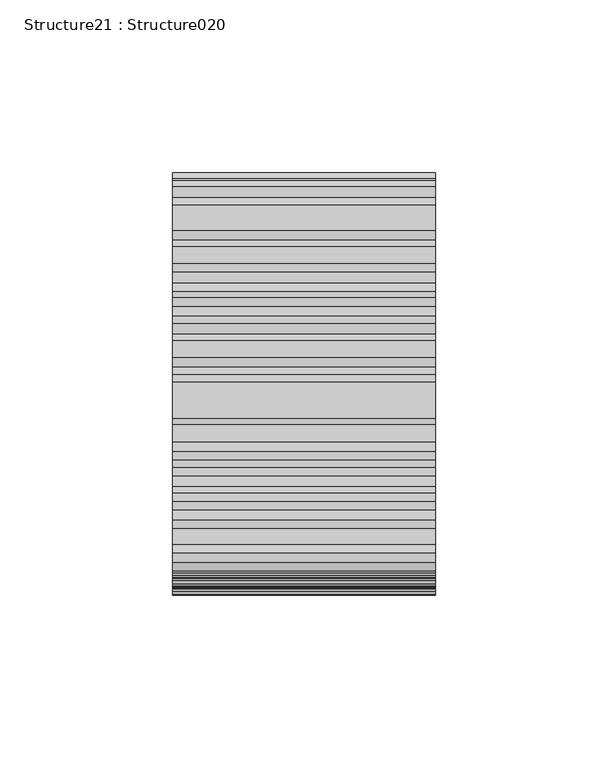
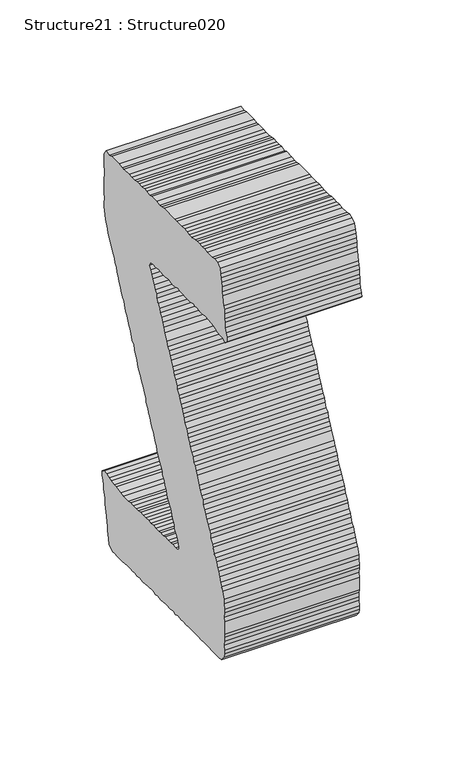
"""IFC4 building model written with IfcOpenShell, lengths in millimetres: proxy geometry, Structure21 : Structure020."""

import ifcopenshell
import ifcopenshell.guid

model = None  # the IFC model being written
_history = None  # IfcOwnerHistory: only IFC2X3 demands one
_inside = {}  # id of a spatial element -> (the spatial element, [elements in it])
_under = {}  # id of a project, library or spatial element -> (it, [spatial elements below it])
_declared = {}  # id of a project -> (the project, [libraries it declares])
_typed = {}  # id of a type object -> (the type object, [elements of that type])
_made_of = {}  # id of a material, layer set ... -> (it, [elements and type objects made of it])


def new_model(schema):
    """Start an empty IFC model of exactly this schema.

    Asked for "IFC4X3", IfcOpenShell would pick the latest addendum, in which some entities
    have other attributes; the version numbers below select the first issue.
    IFC2X3 requires an IfcOwnerHistory on every rooted entity: one is made here for all.
    """
    global model, _history
    if schema == "IFC4X3":
        model = ifcopenshell.file(schema_version=(4, 3, 0, 0))
    else:
        model = ifcopenshell.file(schema=schema)
    _inside.clear()
    _under.clear()
    _declared.clear()
    _typed.clear()
    _made_of.clear()
    _history = None
    if model.schema == "IFC2X3":
        org = make("IfcOrganization", Name="unknown")
        user = make(
            "IfcPersonAndOrganization",
            ThePerson=make("IfcPerson", FamilyName="unknown"),
            TheOrganization=org,
        )
        app = make(
            "IfcApplication",
            ApplicationDeveloper=org,
            Version="unknown",
            ApplicationFullName="unknown",
            ApplicationIdentifier="unknown",
        )
        _history = make(
            "IfcOwnerHistory",
            OwningUser=user,
            OwningApplication=app,
            ChangeAction="ADDED",
            CreationDate=0,
        )
    return model


def make(cls, **values):
    """One entity of the class cls with the attributes given. An attribute that is None is left unset."""
    return model.create_entity(
        cls, **{name: value for name, value in values.items() if value is not None}
    )


def rooted(cls, **values):
    """An entity with a GlobalId (a new one), such as an element, a storey or a relation."""
    return make(cls, GlobalId=ifcopenshell.guid.new(), OwnerHistory=_history, **values)


def si_unit(unit_type, name, prefix=None):
    """IfcSIUnit, for example si_unit("LENGTHUNIT", "METRE", prefix="MILLI")."""
    return make("IfcSIUnit", UnitType=unit_type, Prefix=prefix, Name=name)


def assignment(units):
    """IfcUnitAssignment: the units of a project."""
    return None if units is None else make("IfcUnitAssignment", Units=units)


def point(xyz):
    """IfcCartesianPoint."""
    return None if xyz is None else make("IfcCartesianPoint", Coordinates=xyz)


def direction(xyz):
    """IfcDirection."""
    return None if xyz is None else make("IfcDirection", DirectionRatios=xyz)


def frame(location, z_axis=None, x_axis=None):
    """IfcAxis2Placement3D, a coordinate frame: its origin and axes. An axis left out is left unset."""
    return make(
        "IfcAxis2Placement3D",
        Location=point(location),
        Axis=direction(z_axis),
        RefDirection=direction(x_axis),
    )


def origin():
    """The frame at (0, 0, 0) with its axes left unset."""
    return frame((0.0, 0.0, 0.0))


def place(relative_to, where):
    """IfcLocalPlacement: puts the frame where relative to a parent placement (None: the world)."""
    return make(
        "IfcLocalPlacement", PlacementRelTo=relative_to, RelativePlacement=where
    )


def context(
    kind, dimensions, precision=None, world=None, true_north=None, identifier=None
):
    """IfcGeometricRepresentationContext, for example the 3D "Model" context."""
    return make(
        "IfcGeometricRepresentationContext",
        ContextIdentifier=identifier,
        ContextType=kind,
        CoordinateSpaceDimension=dimensions,
        Precision=precision,
        WorldCoordinateSystem=world,
        TrueNorth=true_north,
    )


def project(units=None, contexts=None):
    """IfcProject with its units and contexts."""
    return rooted(
        "IfcProject",
        Name="project",
        RepresentationContexts=contexts,
        UnitsInContext=assignment(units),
    )


def spatial(cls, under=None, at=None, **own):
    """A site, building, storey or space (cls), placed at a placement, below another one or the project."""
    s = rooted(cls, ObjectPlacement=at, **own)
    if under is not None:
        _under.setdefault(under.id(), (under, []))[1].append(s)
    return s


def polyline(points):
    """IfcPolyline through the points."""
    return make("IfcPolyline", Points=[point(p) for p in points])


def outline(outer, holes=None, kind="AREA"):
    """IfcArbitraryClosedProfileDef: a profile drawn as a closed curve; with holes, ...WithVoids."""
    if holes is None:
        return make("IfcArbitraryClosedProfileDef", ProfileType=kind, OuterCurve=outer)
    return make(
        "IfcArbitraryProfileDefWithVoids",
        ProfileType=kind,
        OuterCurve=outer,
        InnerCurves=holes,
    )


def extrude(swept, where, along, depth):
    """IfcExtrudedAreaSolid: the profile swept, set in the frame where, extruded along a direction by depth."""
    return make(
        "IfcExtrudedAreaSolid",
        SweptArea=swept,
        Position=where,
        ExtrudedDirection=direction(along),
        Depth=depth,
    )


def shape(context_of_items, identifier, shape_type, items):
    """IfcShapeRepresentation: the items that make up one representation, for example the "Body"."""
    return make(
        "IfcShapeRepresentation",
        ContextOfItems=context_of_items,
        RepresentationIdentifier=identifier,
        RepresentationType=shape_type,
        Items=items,
    )


def source(mapping_origin, context_of_items, identifier, shape_type, items):
    """IfcRepresentationMap: a shape defined once, which mapped items show again and again."""
    return make(
        "IfcRepresentationMap",
        MappingOrigin=mapping_origin,
        MappedRepresentation=shape(context_of_items, identifier, shape_type, items),
    )


def transform(
    local_origin,
    x_axis=None,
    y_axis=None,
    z_axis=None,
    scale=None,
    scale2=None,
    scale3=None,
    uniform=True,
):
    """IfcCartesianTransformationOperator3D, or its non-uniform kind. x_axis, y_axis, z_axis: its Axis1, 2, 3."""
    if uniform:
        return make(
            "IfcCartesianTransformationOperator3D",
            Axis1=direction(x_axis),
            Axis2=direction(y_axis),
            LocalOrigin=point(local_origin),
            Scale=scale,
            Axis3=direction(z_axis),
        )
    return make(
        "IfcCartesianTransformationOperator3DnonUniform",
        Axis1=direction(x_axis),
        Axis2=direction(y_axis),
        LocalOrigin=point(local_origin),
        Scale=scale,
        Axis3=direction(z_axis),
        Scale2=scale2,
        Scale3=scale3,
    )


def mapped(mapping_source, mapping_target):
    """IfcMappedItem: shows the shape of a source again, moved by a transform."""
    return make(
        "IfcMappedItem", MappingSource=mapping_source, MappingTarget=mapping_target
    )


def made_of(thing, what):
    """Note that an element or type object is made of a material, layer set ...; save() writes the relation."""
    if what is not None:
        _made_of.setdefault(what.id(), (what, []))[1].append(thing)
    return thing


def element(
    cls,
    number,
    at=None,
    inside=None,
    cuts=None,
    type_object=None,
    material=None,
    context=None,
    identifier="Body",
    shape_type=None,
    held_by="IfcProductDefinitionShape",
    body=None,
    shapes=None,
    **own,
):
    """One element of the class cls, such as IfcWall. Its Tag is "e" and its number.

    at: its placement. inside: the storey or other place that contains it. cuts: it is an
    opening in that element (IfcRelVoidsElement). A single representation is given by context,
    identifier, shape_type and body (its items); several are given by shapes. held_by: the class
    of the entity that holds the representations. save() writes the other relations.
    """
    e = rooted(cls, Tag="e%d" % number, ObjectPlacement=at, **own)
    if body is not None:
        shapes = [shape(context, identifier, shape_type, body)]
    if shapes is not None:
        e.Representation = make(held_by, Representations=shapes)
    if inside is not None:
        _inside.setdefault(inside.id(), (inside, []))[1].append(e)
    if cuts is not None:
        rooted(
            "IfcRelVoidsElement", RelatingBuildingElement=cuts, RelatedOpeningElement=e
        )
    if type_object is not None:
        _typed.setdefault(type_object.id(), (type_object, []))[1].append(e)
    return made_of(e, material)


def aggregate(whole, parts):
    """IfcRelAggregates: a whole, such as a stair, and the parts it consists of."""
    return rooted("IfcRelAggregates", RelatingObject=whole, RelatedObjects=parts)


def save(model, path):
    """Write the relations noted so far, then the file.

    IfcRelAggregates (storeys below a building ...), IfcRelContainedInSpatialStructure (elements
    in a storey), IfcRelDefinesByType, IfcRelAssociatesMaterial and IfcRelDeclares: one each for
    every whole, place, type object, material and project.
    """
    for whole, parts in _under.values():
        aggregate(whole, parts)
    for where, things in _inside.values():
        rooted(
            "IfcRelContainedInSpatialStructure",
            RelatedElements=things,
            RelatingStructure=where,
        )
    for kind, things in _typed.values():
        rooted("IfcRelDefinesByType", RelatedObjects=things, RelatingType=kind)
    for what, things in _made_of.values():
        rooted("IfcRelAssociatesMaterial", RelatedObjects=things, RelatingMaterial=what)
    for by, libraries in _declared.values():
        rooted("IfcRelDeclares", RelatingContext=by, RelatedDefinitions=libraries)
    model.write(path)


def structure21_structure020_0772803a(model_context):
    return source(origin(), model_context, "Body", "SweptSolid", [
        extrude(outline(polyline([(2.4918624, 0.0), (3.6053821, -2.5777483), (4.2923985, -5.0322892), (4.9784696, -7.4834674), (6.2051097, -9.6307181), (6.786362, -12.5115543), (7.588599, -14.5461058), (8.7040111, -17.1169191), (9.3907122, -19.5726158), (10.0484988, -21.3355177), (10.7366711, -23.790374), (11.6968084, -26.099624), (12.9590891, -28.9309487), (14.0327669, -30.8104368), (14.728504, -33.2717039), (15.5358903, -35.3033137), (16.5218964, -38.2914876), (14.6515494, -41.8644896), (12.6100629, -42.6648342), (10.8881597, -44.0143665), (6.0551905, -46.7752522), (1.4453072, -48.6935312), (-0.4349165, -49.7676293), (-2.6987534, -51.4101604), (-5.0008586, -52.3759729), (-6.3008802, -53.8337906), (-8.7605703, -54.5237486), (-11.1382631, -56.5971976), (-16.0151735, -58.6680188), (-20.0426478, -60.9687569), (-21.8811372, -62.7341801), (-24.0738003, -63.2715961), (-26.1837303, -65.1920828), (-28.5980081, -66.571265), (-30.9072573, -67.524572), (-34.9295824, -69.8223685), (-37.4994504, -70.9411433), (-39.0745907, -72.5561256), (-41.2621045, -73.0906), (-43.6361192, -75.1619479), (-45.9453684, -76.1152549), (-48.2101531, -77.774914), (-50.510575, -78.7231783), (-58.5721442, -83.3284365), (-61.1010135, -85.1389568), (-62.8666456, -85.7817167), (-67.4362659, -88.3921614), (-69.4251961, -89.8942357), (-75.6035993, -93.4237151), (-78.4469026, -94.6821062), (-81.7042073, -93.3456045), (-83.4735174, -91.4986033), (-84.542993, -89.6264713), (-85.3862287, -86.9001743), (-86.8885117, -84.900631), (-88.1151519, -82.7533802), (-89.3033146, -81.2934614), (-92.9874372, -74.8443531), (-93.6735083, -72.3931749), (-95.7415992, -70.0231537), (-96.6694586, -68.3989229), (-97.6610341, -65.412955), (-98.8918764, -63.2583482), (-99.9610365, -58.8931981), (-100.0826654, -56.8083995), (-100.076362, -54.3275712), (-100.5013941, -51.711661), (-101.0722447, -48.8404935), (-100.7652682, -46.8757502), (-101.3465204, -43.994914), (-101.8771079, -41.8159121), (-101.3046813, -39.704406), (-102.0318551, -36.5527606), (-102.2714381, -34.9002454), (-101.8835161, -31.8355371), (-102.8382953, -29.5339585), (-102.7960359, -27.7360485), (-103.112571, -24.688379), (-102.8396607, -22.0542732), (-103.1071081, -19.7142173), (-103.1067927, -17.2211991), (-103.1027992, -14.7260798), (-104.2244108, -12.152954), (-103.9102903, -10.2007161), (-104.0675598, -7.4318434), (-104.2165287, -4.6689615), (-104.6456591, 0.4374456), (-104.9040702, 2.7719312), (-105.17614, 5.1200787), (-104.8696903, 7.0737886), (-105.7121904, 9.8005059), (-105.288419, 12.1705271), (-105.4456884, 14.9393997), (-105.9808984, 17.1264933), (-105.9763807, 19.6121554), (-106.0908657, 21.6844485), (-106.515689, 24.2897458), (-106.3975243, 27.2169388), (-106.8219272, 29.8215003), (-106.9398781, 31.9084001), (-107.6340409, 34.3549557), (-107.6252136, 36.8518608), (-107.7822742, 39.6101204), (-108.0081977, 41.2558037), (-107.6286802, 44.3352243), (-108.2712313, 46.0902433), (-108.3147513, 49.2782648), (-108.1680933, 51.5065685), (-108.6996253, 53.6957631), (-108.9704352, 56.0348738), (-109.0023977, 59.2129112), (-109.2814025, 61.5629511), (-109.6960329, 64.1691928), (-109.117828, 66.2722918), (-109.9631649, 69.0022668), (-109.9194334, 73.2997099), (-110.0806962, 76.0653255), (-110.9193095, 78.7835307), (-110.9189941, 81.276549), (-110.4998452, 83.654662), (-111.4550446, 85.9569761), (-111.4618729, 88.4624997), (-111.1841288, 91.0983913), (-112.1520425, 93.4041746), (-111.8404434, 95.3608262), (-112.2650553, 97.9760009), (-112.144896, 100.8877469), (-112.4163368, 103.2245458), (-112.261587, 105.4574719), (-112.2557038, 107.9390358), (-114.8300877, 109.331984), (-117.2886221, 108.6417106), (-119.3989723, 106.7219595), (-121.8545642, 106.033367), (-123.7340522, 104.9596892), (-125.5773754, 103.1924802), (-127.4575991, 102.1183821), (-130.1831605, 101.2755667), (-131.6454959, 100.0899261), (-133.6315885, 98.5914242), (-136.053958, 97.2076195), (-138.2410517, 96.6724096), (-139.9704141, 95.3342269), (-142.6561326, 93.7999813), (-144.1074355, 92.6069838), (-148.6814695, 89.9940177), (-151.3996747, 89.1554045), (-152.4360318, 87.8491835), (-155.1630644, 87.0055276), (-157.0063876, 85.2383185), (-158.8866113, 84.1642205), (-161.8799354, 83.1684427), (-163.4518178, 81.5562971), (-167.2107939, 79.4089415), (-169.2837179, 76.8002825), (-170.8530791, 75.1837233), (-172.8543025, 73.6912129), (-174.5737892, 72.3391585), (-176.1190672, 70.0485093), (-178.9153839, 70.5780449), (-179.8744701, 72.888871), (-180.1426531, 75.2285067), (-180.8312455, 77.6840985), (-182.1014065, 80.5206782), (-182.7532027, 82.2918807), (-184.2807247, 84.9658294), (-185.2470613, 87.277392), (-185.6218497, 89.1853733), (-187.4306864, 94.2236531), (-187.9661078, 96.4008692), (-189.354535, 98.8313304), (-190.3085786, 101.1333292), (-190.9990633, 103.581986), (-191.3830967, 105.5061509), (-192.372151, 108.4877051), (-191.1508672, 111.3455109), (-189.0399927, 113.2558048), (-186.5900743, 113.9509129), (-182.5581863, 116.2541724), (-180.7150744, 118.011504), (-178.1441563, 119.1250246), (-176.1454543, 120.6219487), (-174.0018816, 121.8464877), (-172.2320446, 122.502382), (-169.3966208, 123.7728584), (-167.2449564, 125.0020198), (-165.5159093, 126.3390467), (-163.5260346, 127.8309281), (-160.9499672, 128.9473903), (-156.6554658, 131.4006705), (-155.192289, 132.59167), (-146.065554, 137.8054156), (-144.0331036, 138.6113307), (-141.998761, 139.4241808), (-139.8834728, 141.3369961), (-135.589707, 143.789856), (-133.6738428, 144.17988), (-131.2871138, 146.2477587), (-129.4068902, 147.3218567), (-126.8403857, 148.432856), (-124.8416837, 149.9297801), (-123.2292227, 150.8509158), (-120.7793043, 151.5460239), (-118.0928502, 153.0806898), (-116.0916267, 154.5732003), (-111.797861, 157.0260602), (-110.0393727, 157.6813255), (-107.9204065, 159.5962419), (-101.4742407, 163.2786835), (-99.2913493, 163.8212496), (-96.905356, 165.8887081), (-93.9075143, 164.3864232), (-92.5679653, 162.6597927), (-91.4504521, 160.0853013), (-90.3830777, 158.2168475), (-89.4290342, 155.9148487), (-88.0406071, 153.4843874), (-86.4326637, 151.919861), (-85.2081248, 149.7762884), (-84.0838879, 147.1900273), (-82.5981002, 145.2074038), (-81.8269853, 143.8575563), (-81.1417546, 141.4078493), (-79.2194821, 139.2930853), (-78.1011284, 136.7171227), (-77.459313, 134.9616834), (-75.9577663, 130.4630273), (-75.6938923, 125.6271165), (-74.7342784, 123.3341538), (-74.6943316, 120.1421398), (-74.5837334, 118.0783585), (-74.8450879, 115.4206082), (-74.5808984, 113.0777156), (-74.5760646, 110.587639), (-73.8914646, 108.1356203), (-74.315236, 105.7655992), (-73.3558344, 103.4559288), (-73.3118941, 100.2671717), (-72.9281762, 98.3418511), (-72.7777352, 95.5866397), (-72.6651425, 93.5074115), (-72.3564851, 90.4854876), (-72.9383681, 88.3802874), (-72.1253092, 86.3353317), (-71.8255839, 83.3102565), (-72.2454685, 80.9317233), (-71.977601, 78.5909318), (-71.550888, 75.9720791), (-71.4003422, 73.2149762), (-70.443987, 68.4204844), (-71.2924768, 66.1620065), (-70.5971599, 63.701475), (-70.3292923, 61.3606835), (-70.2899745, 58.1800181), (-69.9073067, 56.2599516), (-69.4880529, 53.6524485), (-69.7544509, 50.9966953), (-69.3719919, 49.087242), (-69.3759853, 46.5921226), (-69.3758805, 44.0983688), (-68.9464347, 41.4849799), (-69.2174553, 38.8373185), (-68.4159538, 36.8023468), (-68.6480768, 33.4666179), (-68.1099243, 31.2812053), (-68.104146, 28.7809358), (-67.9514991, 26.0201549), (-67.6884654, 23.6775777), (-67.8415317, 21.4621997), (-67.2635374, 18.5785267), (-67.2675308, 16.0834073), (-67.0424477, 14.4391952), (-66.7634429, 12.0891554), (-66.309914, 8.8016765), (-66.5737907, 6.1415096), (-66.3059232, 1.3088558), (-65.6571727, -0.4484758), (-66.040681, -3.5106627), (-65.5031611, -5.7120475), (-65.7700833, -8.3583433), (-64.8116261, -10.6578208), (-64.5481723, -13.0011336), (-64.9669009, -17.8718446), (-64.3960504, -20.7430121), (-64.2366799, -23.5155628), (-64.2399377, -26.0102619), (-63.4291887, -28.0409264), (-63.821209, -31.1070004), (-63.8530667, -32.914579), (-63.2858942, -35.7878477), (-62.8935602, -37.7180031), (-61.4415217, -39.0164477), (-58.8710238, -37.9021914), (-56.6011963, -36.2513597), (-54.5684307, -35.4442888), (-52.4263292, -34.2205902), (-50.1594442, -32.5714394), (-47.9661512, -32.038542), (-45.9801634, -30.5381486), (-44.2064395, -29.8907662), (-41.9497466, -28.2357296), (-40.2183869, -26.8925034), (-37.221806, -25.9007191), (-35.9202075, -24.4371221), (-33.3533876, -23.324967), (-31.2017232, -22.0958055), (-29.2077503, -20.6025586), (-26.7496369, -19.9183798), (-25.2954965, -18.7218099), (-22.4477795, -17.4608974), (-20.8776827, -15.8439178), (-18.4210407, -15.1605795), (-14.1228612, -12.7051982), (-12.2813238, -10.9331553), (-8.5670244, -8.0961554), (-7.1034275, -6.9058915), (-4.5741379, -5.0961068), (-3.2648714, -3.6544726), (-1.9987022, -1.4969241), (0.0, 0.0), (2.4918624, 0.0)])), frame((-35624.0862846, 275354.7652277, 4026.4392678), z_axis=(1.0, 0.0, 1.3542500454377661e-12), x_axis=(0.0, 0.8683059004905059, -0.496029095087548)), (0.0, 0.0, 1.0), 76.2),
    ])


if __name__ == "__main__":
    model = new_model("IFC4")
    model_context = context("Model", 3, world=origin())
    ifc_project = project(units=[si_unit("LENGTHUNIT", "METRE", prefix="MILLI")], contexts=[model_context])
    site = spatial("IfcSite", under=ifc_project)
    building = spatial("IfcBuilding", under=site)
    placement = place(None, origin())
    structure21_structure020_shape = structure21_structure020_0772803a(model_context)
    element("IfcBuildingElementProxy", 1, Name="Structure21 : Structure020", ObjectType="Structure21 : Structure020", at=placement, inside=building, context=model_context, shape_type="MappedRepresentation", body=[
        mapped(structure21_structure020_shape, transform((0.0, 0.0, 0.0), x_axis=(1.0, 0.0, 0.0), y_axis=(0.0, 1.0, 0.0), z_axis=(0.0, 0.0, 1.0))),
    ])
    save(model, "model.ifc")

# Revit data of these elements
# Type "Structure21 : Structure020"
#   NameOverride = "Structure020"
# Element 1 (IfcBuildingElementProxy, "Structure21 : Structure020")
#   Materials on its faces: "BRUSHED ALUMINUM LETTERING"
# Materials
#   "BRUSHED ALUMINUM LETTERING": class "Unassigned", colour RGB 169 181 186, transparency 0, Cost = 0
